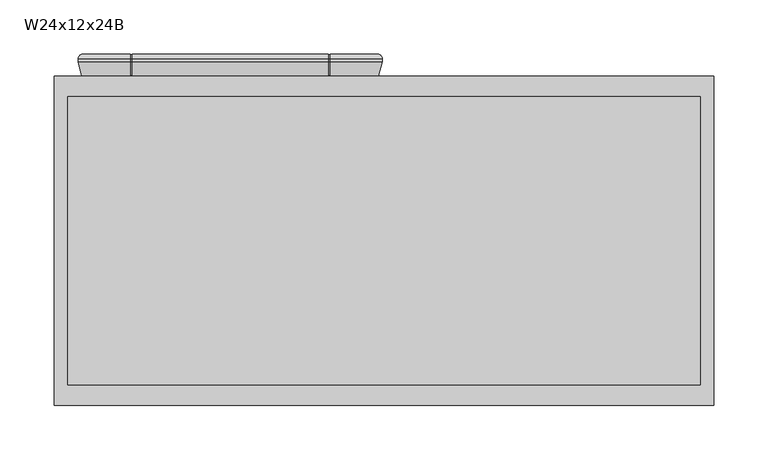
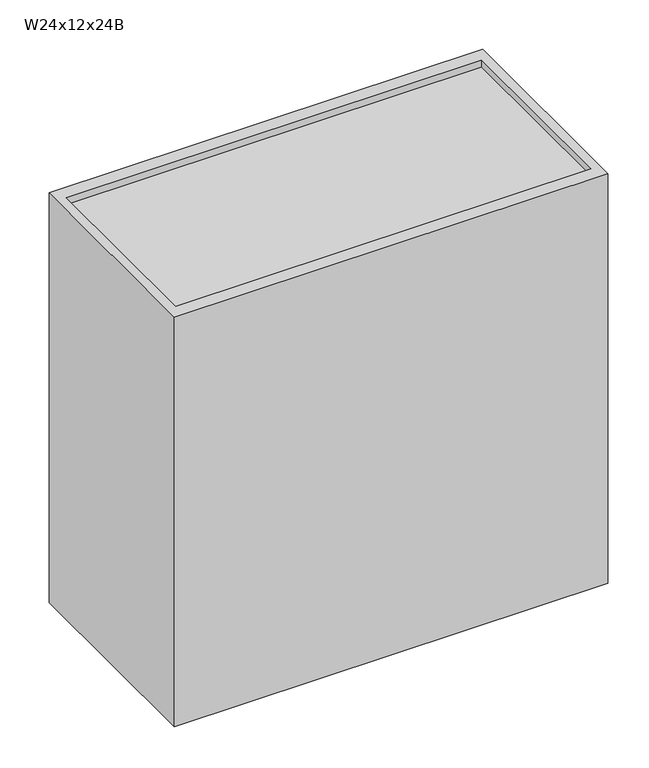
"""IFC4 building model written with IfcOpenShell, lengths in millimetres: furniture geometry, Cabinet-Wall-Merillat-Double_Door-Marlin : W24x12x24B."""

from ifc_helpers import new_model, si_unit, frame, origin, place, context, project, spatial, polyline, circle_curve, ellipse_curve, outline, extrude, faceted_brep, source, transform, mapped, element, save
from ifc_brep_helpers import plane_surface, cylinder_surface, advanced_brep


def w24x12x24b_bf14e69a(model_context):
    return source(origin(), model_context, "Body", "SolidModel", [
        advanced_brep(
        [(-24.0971608, 382.5621, 2108.2), (-21.0006683, 387.0325, 2105.1035075), (-21.0006683, 387.0325, 1552.4964925), (-24.0971608, 382.5621, 1549.4), (-24.0971608, 379.7935, 1549.4), (-24.0971608, 379.7935, 2108.2), (-20.5919608, 366.7125, 1552.9052), (-20.5919608, 366.7125, 2104.6948), (24.104002, 366.7125, 2059.9988372), (24.104002, 366.7125, 1597.6011628), (24.4741337, 367.50625, 1597.9712945), (26.5552927, 371.96931, 1600.0524535), (26.5552927, 371.96931, 2057.5475465), (24.4741337, 367.50625, 2059.6287055), (25.1555233, 374.2094093, 1598.652684), (25.1555233, 374.2094093, 2058.947316), (10.8278392, 374.4595, 1584.325), (10.8278392, 374.4595, 2073.275), (10.8278392, 379.2855, 1584.325), (10.8278392, 379.2855, 2073.275), (25.1555233, 379.5355907, 1598.652684), (25.1555233, 379.5355907, 2058.947316), (26.5552927, 381.77569, 1600.0524535), (26.5552927, 381.77569, 2057.5475465), (24.4741337, 386.23875, 1597.9712945), (24.1068694, 387.0263508, 1597.6040302), (24.104002, 387.0325, 2059.9988372), (24.4741337, 386.23875, 2059.6287055), (24.1068694, 387.0325, 1552.4964925), (24.1068694, 382.5621, 1549.4), (253.7938467, 387.0325, 1552.4964925), (256.8903392, 382.5621, 1549.4), (208.7261206, 382.5621, 1549.4), (208.7261206, 387.0325, 1552.4964925), (25.6943694, 382.5621, 1549.4), (25.6943694, 387.0325, 1552.4964925), (207.1386206, 387.0325, 1552.4964925), (207.1386206, 382.5621, 1549.4), (24.1068694, 379.7935, 1549.4), (256.8903392, 379.7935, 1549.4), (208.7261206, 379.7935, 1549.4), (25.6943694, 379.7935, 1549.4), (207.1386206, 379.7935, 1549.4), (24.1068694, 366.7125, 1552.9052), (253.3851392, 366.7125, 1552.9052), (208.7261206, 366.7125, 1552.9052), (25.6943694, 366.7125, 1552.9052), (207.1386206, 366.7125, 1552.9052), (206.2378857, 371.96931, 1600.0524535), (25.6943694, 367.50625, 1597.9712945), (25.6943694, 366.7125, 1597.6011628), (207.1386206, 366.7125, 1597.6011628), (207.1386206, 367.50625, 1597.9712945), (208.3190448, 367.50625, 1597.9712945), (207.6376552, 374.2094093, 1598.652684), (221.9653392, 374.4595, 1584.325), (221.9653392, 379.2855, 1584.325), (207.6376552, 379.5355907, 1598.652684), (206.2378857, 381.77569, 1600.0524535), (208.3190448, 386.23875, 1597.9712945), (207.1386206, 386.23875, 1597.9712945), (207.1386206, 387.0325, 1597.6011628), (25.6943694, 387.0325, 1597.6011628), (25.6943694, 386.23875, 1597.9712945), (253.7938467, 387.0325, 2105.1035075), (256.8903392, 382.5621, 2108.2), (256.8903392, 379.7935, 2108.2), (253.3851392, 366.7125, 2104.6948), (208.6891765, 366.7125, 1597.6011628), (208.6891765, 366.7125, 2059.9988372), (208.3190448, 367.50625, 2059.6287055), (206.2378857, 371.96931, 2057.5475465), (207.6376552, 374.2094093, 2058.947316), (221.9653392, 374.4595, 2073.275), (221.9653392, 379.2855, 2073.275), (207.6376552, 379.5355907, 2058.947316), (206.2378857, 381.77569, 2057.5475465), (208.3190448, 386.23875, 2059.6287055), (208.6891765, 387.0325, 2059.9988372), (208.6891765, 387.0325, 1597.6011628), (208.7261206, 387.0325, 2105.1035075), (208.7261206, 382.5621, 2108.2), (24.1068694, 382.5621, 2108.2), (24.1068694, 387.0325, 2105.1035075), (207.1386206, 382.5621, 2108.2), (207.1386206, 387.0325, 2105.1035075), (25.6943694, 387.0325, 2105.1035075), (25.6943694, 382.5621, 2108.2), (208.7261206, 379.7935, 2108.2), (24.1068694, 379.7935, 2108.2), (207.1386206, 379.7935, 2108.2), (25.6943694, 379.7935, 2108.2), (208.7261206, 366.7125, 2104.6948), (24.1068694, 366.7125, 2104.6948), (207.1386206, 366.7125, 2104.6948), (25.6943694, 366.7125, 2104.6948), (207.1386206, 366.7125, 2059.9988372), (25.6943694, 366.7125, 2059.9988372), (207.1386206, 367.50625, 2059.6287055), (25.6943694, 367.50625, 2059.6287055), (25.6943694, 386.23875, 2059.6287055), (25.6943694, 387.0325, 2059.9988372), (207.1386206, 387.0325, 2059.9988372), (207.1386206, 386.23875, 2059.6287055), (207.1386206, 367.50625, 2104.0857412), (207.1386206, 379.8980037, 2107.40625), (207.1386206, 382.5621, 2107.40625), (207.1386206, 386.23875, 2104.9526052), (208.7261206, 386.23875, 2059.6287055), (208.7261206, 386.23875, 2104.9526052), (208.7261206, 382.5621, 2107.40625), (208.7261206, 379.8980037, 2107.40625), (208.7261206, 367.50625, 2104.0857412), (208.7261206, 367.50625, 2059.6287055), (24.1068694, 367.50625, 2059.6287055), (24.1068694, 367.50625, 2104.0857412), (24.1068694, 379.8980037, 2107.40625), (24.1068694, 382.5621, 2107.40625), (24.1068694, 386.23875, 2104.9526052), (24.1068694, 386.23875, 2059.6287055), (25.6943694, 386.23875, 2104.9526052), (25.6943694, 382.5621, 2107.40625), (25.6943694, 379.8980037, 2107.40625), (25.6943694, 367.50625, 2104.0857412), (24.1068694, 386.23875, 1597.9712945), (24.1068694, 386.23875, 1552.6473948), (24.1068694, 382.5621, 1550.19375), (24.1068694, 379.8980037, 1550.19375), (24.1068694, 367.50625, 1553.5142588), (24.1068694, 367.50625, 1597.9712945), (25.6943694, 367.50625, 1553.5142588), (25.6943694, 379.8980037, 1550.19375), (25.6943694, 382.5621, 1550.19375), (25.6943694, 386.23875, 1552.6473948), (207.1386206, 386.23875, 1552.6473948), (207.1386206, 382.5621, 1550.19375), (207.1386206, 379.8980037, 1550.19375), (207.1386206, 367.50625, 1553.5142588), (208.7261206, 386.23875, 1597.9712945), (208.7261206, 367.50625, 1597.9712945), (208.7261206, 367.50625, 1553.5142588), (208.7261206, 379.8980037, 1550.19375), (208.7261206, 382.5621, 1550.19375), (208.7261206, 386.23875, 1552.6473948)],
        [
            (0, 1, ellipse_curve(frame((-19.3219608, 382.5621, 2103.4248), z_axis=(-0.7071067811865475, 0.0, -0.7071067811865475), x_axis=(-0.7071067811865474, 0.0, 0.7071067811865476)), 6.7531526, 4.7752)),
            (1, 2),
            (2, 3, ellipse_curve(frame((-19.3219608, 382.5621, 1554.1752), z_axis=(-0.7071067811865475, 0.0, 0.7071067811865475), x_axis=(0.7071067811865474, 0.0, 0.7071067811865476)), 6.7531526, 4.7752)),
            (3, 0),
            (3, 4),
            (4, 5),
            (5, 0),
            (4, 6),
            (6, 7),
            (7, 5),
            (8, 9),
            (9, 10),
            (10, 11),
            (11, 12),
            (12, 13),
            (13, 8),
            (11, 14, ellipse_curve(frame((25.1280392, 372.6348492, 1598.6252), z_axis=(-0.7071067811865475, 0.0, 0.7071067811865475), x_axis=(0.7071067811865474, 0.0, 0.7071067811865476)), 2.2271035, 1.5748)),
            (14, 15),
            (15, 12, ellipse_curve(frame((25.1280392, 372.6348492, 2058.9748), z_axis=(-0.7071067811865475, 0.0, -0.7071067811865475), x_axis=(-0.7071067811865474, 0.0, 0.7071067811865476)), 2.2271035, 1.5748)),
            (14, 16),
            (16, 17),
            (17, 15),
            (16, 18),
            (18, 19),
            (19, 17),
            (18, 20),
            (20, 21),
            (21, 19),
            (20, 22, ellipse_curve(frame((25.1280392, 381.1101508, 1598.6252), z_axis=(-0.7071067811865475, 0.0, 0.7071067811865475), x_axis=(0.7071067811865474, 0.0, 0.7071067811865476)), 2.2271035, 1.5748)),
            (22, 23),
            (23, 21, ellipse_curve(frame((25.1280392, 381.1101508, 2058.9748), z_axis=(-0.7071067811865475, 0.0, -0.7071067811865475), x_axis=(-0.7071067811865474, 0.0, 0.7071067811865476)), 2.2271035, 1.5748)),
            (22, 24),
            (24, 25),
            (25, 26),
            (26, 27),
            (27, 23),
            (2, 28),
            (28, 29, circle_curve(frame((24.1068694, 382.5621, 1554.1752), z_axis=(-1.0, 0.0, 0.0), x_axis=(0.0, -1.0, 0.0)), 4.7752)),
            (29, 3),
            (30, 31, ellipse_curve(frame((252.1151392, 382.5621, 1554.1752), z_axis=(-0.7071067811865475, 0.0, -0.7071067811865475), x_axis=(-0.7071067811865476, 0.0, 0.7071067811865474)), 6.7531526, 4.7752)),
            (31, 32),
            (32, 33, circle_curve(frame((208.7261206, 382.5621, 1554.1752), z_axis=(1.0, 0.0, 0.0), x_axis=(0.0, -1.0, 0.0)), 4.7752)),
            (33, 30),
            (34, 35, circle_curve(frame((25.6943694, 382.5621, 1554.1752), z_axis=(1.0, 0.0, 0.0), x_axis=(0.0, -1.0, 0.0)), 4.7752)),
            (35, 36),
            (36, 37, circle_curve(frame((207.1386206, 382.5621, 1554.1752), z_axis=(-1.0, 0.0, 0.0), x_axis=(0.0, -1.0, 0.0)), 4.7752)),
            (37, 34),
            (29, 38),
            (38, 4),
            (31, 39),
            (39, 40),
            (40, 32),
            (41, 34),
            (37, 42),
            (42, 41),
            (38, 43),
            (43, 6),
            (39, 44),
            (44, 45),
            (45, 40),
            (46, 41),
            (42, 47),
            (47, 46),
            (48, 11),
            (10, 49),
            (49, 50),
            (50, 51),
            (51, 52),
            (52, 53),
            (53, 48),
            (48, 54, ellipse_curve(frame((207.6651392, 372.6348492, 1598.6252), z_axis=(-0.7071067811865475, 0.0, -0.7071067811865475), x_axis=(-0.7071067811865476, 0.0, 0.7071067811865474)), 2.2271035, 1.5748)),
            (54, 14),
            (54, 55),
            (55, 16),
            (55, 56),
            (56, 18),
            (56, 57),
            (57, 20),
            (57, 58, ellipse_curve(frame((207.6651392, 381.1101508, 1598.6252), z_axis=(-0.7071067811865475, 0.0, -0.7071067811865475), x_axis=(-0.7071067811865476, 0.0, 0.7071067811865474)), 2.2271035, 1.5748)),
            (58, 22),
            (58, 59),
            (59, 60),
            (60, 61),
            (61, 62),
            (62, 63),
            (63, 24),
            (30, 64),
            (64, 65, ellipse_curve(frame((252.1151392, 382.5621, 2103.4248), z_axis=(0.7071067811865475, 0.0, -0.7071067811865475), x_axis=(-0.7071067811865474, 0.0, -0.7071067811865476)), 6.7531526, 4.7752)),
            (65, 31),
            (65, 66),
            (66, 39),
            (66, 67),
            (67, 44),
            (68, 69),
            (69, 70),
            (70, 71),
            (71, 48),
            (53, 68),
            (71, 72, ellipse_curve(frame((207.6651392, 372.6348492, 2058.9748), z_axis=(0.7071067811865475, 0.0, -0.7071067811865475), x_axis=(-0.7071067811865474, 0.0, -0.7071067811865476)), 2.2271035, 1.5748)),
            (72, 54),
            (72, 73),
            (73, 55),
            (73, 74),
            (74, 56),
            (74, 75),
            (75, 57),
            (75, 76, ellipse_curve(frame((207.6651392, 381.1101508, 2058.9748), z_axis=(0.7071067811865475, 0.0, -0.7071067811865475), x_axis=(-0.7071067811865474, 0.0, -0.7071067811865476)), 2.2271035, 1.5748)),
            (76, 58),
            (76, 77),
            (77, 78),
            (78, 79),
            (79, 59),
            (64, 80),
            (80, 81, circle_curve(frame((208.7261206, 382.5621, 2103.4248), z_axis=(1.0, 0.0, 0.0), x_axis=(0.0, -1.0, 0.0)), 4.7752)),
            (81, 65),
            (0, 82),
            (82, 83, circle_curve(frame((24.1068694, 382.5621, 2103.4248), z_axis=(-1.0, 0.0, 0.0), x_axis=(0.0, -1.0, 0.0)), 4.7752)),
            (83, 1),
            (84, 85, circle_curve(frame((207.1386206, 382.5621, 2103.4248), z_axis=(-1.0, 0.0, 0.0), x_axis=(0.0, -1.0, 0.0)), 4.7752)),
            (85, 86),
            (86, 87, circle_curve(frame((25.6943694, 382.5621, 2103.4248), z_axis=(1.0, 0.0, 0.0), x_axis=(0.0, -1.0, 0.0)), 4.7752)),
            (87, 84),
            (81, 88),
            (88, 66),
            (5, 89),
            (89, 82),
            (90, 84),
            (87, 91),
            (91, 90),
            (88, 92),
            (92, 67),
            (7, 93),
            (93, 89),
            (94, 90),
            (91, 95),
            (95, 94),
            (43, 9),
            (8, 93),
            (92, 69),
            (68, 45),
            (96, 94),
            (95, 97),
            (97, 96),
            (50, 46),
            (47, 51),
            (12, 71),
            (70, 98),
            (98, 96),
            (97, 99),
            (99, 13),
            (15, 72),
            (17, 73),
            (19, 74),
            (21, 75),
            (23, 76),
            (27, 100),
            (100, 101),
            (101, 102),
            (102, 103),
            (103, 77),
            (83, 26),
            (25, 28),
            (33, 79),
            (78, 80),
            (85, 102),
            (101, 86),
            (35, 62),
            (61, 36),
            (98, 104),
            (104, 105),
            (105, 106),
            (106, 107, circle_curve(frame((207.1386206, 382.5621, 2103.4248), z_axis=(-1.0, 0.0, 0.0), x_axis=(0.0, 0.0, 1.0)), 3.98145)),
            (107, 103),
            (78, 108),
            (108, 109),
            (109, 110, circle_curve(frame((208.7261206, 382.5621, 2103.4248), z_axis=(1.0, 0.0, 0.0), x_axis=(0.0, 0.0, 1.0)), 3.98145)),
            (110, 111),
            (111, 112),
            (112, 113),
            (113, 69),
            (77, 108),
            (107, 109),
            (106, 110),
            (105, 111),
            (104, 112),
            (70, 113),
            (8, 114),
            (114, 115),
            (115, 116),
            (116, 117),
            (117, 118, circle_curve(frame((24.1068694, 382.5621, 2103.4248), z_axis=(-1.0, 0.0, 0.0), x_axis=(0.0, 0.0, 1.0)), 3.98145)),
            (118, 119),
            (119, 26),
            (100, 120),
            (120, 121, circle_curve(frame((25.6943694, 382.5621, 2103.4248), z_axis=(1.0, 0.0, 0.0), x_axis=(0.0, 0.0, 1.0)), 3.98145)),
            (121, 122),
            (122, 123),
            (123, 99),
            (119, 27),
            (118, 120),
            (117, 121),
            (116, 122),
            (115, 123),
            (114, 13),
            (25, 124),
            (124, 125),
            (125, 126, circle_curve(frame((24.1068694, 382.5621, 1554.1752), z_axis=(-1.0, 0.0, 0.0), x_axis=(0.0, 0.0, 1.0)), 3.98145)),
            (126, 127),
            (127, 128),
            (128, 129),
            (129, 9),
            (49, 130),
            (130, 131),
            (131, 132),
            (132, 133, circle_curve(frame((25.6943694, 382.5621, 1554.1752), z_axis=(1.0, 0.0, 0.0), x_axis=(0.0, 0.0, 1.0)), 3.98145)),
            (133, 63),
            (129, 10),
            (128, 130),
            (127, 131),
            (126, 132),
            (125, 133),
            (124, 24),
            (60, 134),
            (134, 135, circle_curve(frame((207.1386206, 382.5621, 1554.1752), z_axis=(-1.0, 0.0, 0.0), x_axis=(0.0, 0.0, 1.0)), 3.98145)),
            (135, 136),
            (136, 137),
            (137, 52),
            (138, 79),
            (68, 139),
            (139, 140),
            (140, 141),
            (141, 142),
            (142, 143, circle_curve(frame((208.7261206, 382.5621, 1554.1752), z_axis=(1.0, 0.0, 0.0), x_axis=(0.0, 0.0, 1.0)), 3.98145)),
            (143, 138),
            (138, 59),
            (53, 139),
            (137, 140),
            (136, 141),
            (135, 142),
            (134, 143),
        ],
        [
            cylinder_surface(frame((-19.3219608, 382.5621, 2108.2), z_axis=(0.0, 0.0, 1.0), x_axis=(0.0, -1.0, 0.0)), 4.7752),
            plane_surface(frame((-24.0971608, 382.5621, 2108.2), z_axis=(-1.0, 0.0, 0.0), x_axis=(0.0, 0.0, -1.0))),
            plane_surface(frame((-24.0971608, 379.7935, 2108.2), z_axis=(-0.9659229350723619, -0.25882983502910506, 0.0), x_axis=(0.0, 0.0, -1.0))),
            plane_surface(frame((24.104002, 366.7125, 2059.9988372), z_axis=(0.9063077870366099, -0.4226182617407856, 0.0), x_axis=(0.0, 0.0, -1.0))),
            cylinder_surface(frame((25.1280392, 372.6348492, 2108.2), z_axis=(0.0, 0.0, 1.0000000000000002), x_axis=(0.01745240643729364, 0.9998476951563912, 0.0)), 1.5748),
            plane_surface(frame((25.1555233, 374.2094093, 2058.947316), z_axis=(0.017452406437322144, 0.9998476951563906, 0.0), x_axis=(0.0, 0.0, -1.0))),
            plane_surface(frame((10.8278392, 374.4595, 2073.275), z_axis=(1.0, 0.0, 0.0), x_axis=(0.0, 0.0, -1.0))),
            plane_surface(frame((10.8278392, 379.2855, 2073.275), z_axis=(0.01745240643727848, -0.9998476951563914, 0.0), x_axis=(0.0, 0.0, -1.0))),
            cylinder_surface(frame((25.1280392, 381.1101508, 2108.2), z_axis=(0.0, 0.0, 1.0000000000000002), x_axis=(0.9063077870367326, 0.42261826174052236, 0.0)), 1.5748),
            plane_surface(frame((26.5552927, 381.77569, 2057.5475465), z_axis=(0.9063077870366333, 0.4226182617407352, 0.0), x_axis=(0.0, 0.0, -1.0))),
            cylinder_surface(frame((-24.0971608, 382.5621, 1554.1752), z_axis=(-1.0, 0.0, 0.0), x_axis=(0.0, -1.0, 0.0)), 4.7752),
            plane_surface(frame((-24.0971608, 382.5621, 1549.4), z_axis=(0.0, 0.0, -1.0), x_axis=(1.0, 0.0, 0.0))),
            plane_surface(frame((-24.0971608, 379.7935, 1549.4), z_axis=(0.0, -0.2588298350291095, -0.9659229350723607), x_axis=(1.0, 0.0, 0.0))),
            plane_surface(frame((24.104002, 366.7125, 1597.6011628), z_axis=(0.0, -0.42261826174078143, 0.9063077870366119), x_axis=(1.0, 0.0, 0.0))),
            cylinder_surface(frame((-24.0971608, 372.6348492, 1598.6252), z_axis=(-1.0000000000000002, 0.0, 0.0), x_axis=(0.0, 0.9998476951563913, 0.017452406437289025)), 1.5748),
            plane_surface(frame((25.1555233, 374.2094093, 1598.652684), z_axis=(0.0, 0.9998476951563907, 0.01745240643731753), x_axis=(1.0, 0.0, 0.0))),
            plane_surface(frame((10.8278392, 374.4595, 1584.325), z_axis=(0.0, 0.0, 1.0), x_axis=(1.0, 0.0, 0.0))),
            plane_surface(frame((10.8278392, 379.2855, 1584.325), z_axis=(0.0, -0.9998476951563913, 0.017452406437283095), x_axis=(1.0, 0.0, 0.0))),
            cylinder_surface(frame((-24.0971608, 381.1101508, 1598.6252), z_axis=(-1.0000000000000002, 0.0, 0.0), x_axis=(0.0, 0.4226182617405265, 0.9063077870367306)), 1.5748),
            plane_surface(frame((26.5552927, 381.77569, 1600.0524535), z_axis=(0.0, 0.4226182617407394, 0.9063077870366314), x_axis=(1.0, 0.0, 0.0))),
            cylinder_surface(frame((252.1151392, 382.5621, 1549.4), z_axis=(0.0, 0.0, -1.0), x_axis=(0.0, -1.0, 0.0)), 4.7752),
            plane_surface(frame((256.8903392, 382.5621, 1549.4), z_axis=(1.0, 0.0, 0.0), x_axis=(0.0, 0.0, 1.0))),
            plane_surface(frame((256.8903392, 379.7935, 1549.4), z_axis=(0.9659229350723619, -0.25882983502910506, 0.0), x_axis=(0.0, 0.0, 1.0))),
            plane_surface(frame((208.6891765, 366.7125, 1597.6011628), z_axis=(-0.9063077870366099, -0.4226182617407856, 0.0), x_axis=(0.0, 0.0, 1.0))),
            cylinder_surface(frame((207.6651392, 372.6348492, 1549.4), z_axis=(0.0, 0.0, -1.0000000000000002), x_axis=(-0.01745240643729364, 0.9998476951563912, 0.0)), 1.5748),
            plane_surface(frame((207.6376552, 374.2094093, 1598.652684), z_axis=(-0.017452406437322144, 0.9998476951563906, 0.0), x_axis=(0.0, 0.0, 1.0))),
            plane_surface(frame((221.9653392, 374.4595, 1584.325), z_axis=(-1.0, 0.0, 0.0), x_axis=(0.0, 0.0, 1.0))),
            plane_surface(frame((221.9653392, 379.2855, 1584.325), z_axis=(-0.01745240643727848, -0.9998476951563914, 0.0), x_axis=(0.0, 0.0, 1.0))),
            cylinder_surface(frame((207.6651392, 381.1101508, 1549.4), z_axis=(0.0, 0.0, -1.0000000000000002), x_axis=(-0.9063077870367326, 0.42261826174052236, 0.0)), 1.5748),
            plane_surface(frame((206.2378857, 381.77569, 1600.0524535), z_axis=(-0.9063077870366333, 0.4226182617407352, 0.0), x_axis=(0.0, 0.0, 1.0))),
            cylinder_surface(frame((256.8903392, 382.5621, 2103.4248), z_axis=(1.0, 0.0, 0.0), x_axis=(0.0, -1.0, 0.0)), 4.7752),
            plane_surface(frame((256.8903392, 382.5621, 2108.2), z_axis=(0.0, 0.0, 1.0), x_axis=(-1.0, 0.0, 0.0))),
            plane_surface(frame((256.8903392, 379.7935, 2108.2), z_axis=(0.0, -0.2588298350291006, 0.9659229350723632), x_axis=(-1.0, 0.0, 0.0))),
            plane_surface(frame((253.3851392, 366.7125, 2104.6948), z_axis=(0.0, -1.0, 0.0), x_axis=(-1.0, 0.0, 0.0))),
            plane_surface(frame((208.6891765, 366.7125, 2059.9988372), z_axis=(0.0, -0.42261826174078976, -0.9063077870366079), x_axis=(-1.0, 0.0, 0.0))),
            cylinder_surface(frame((256.8903392, 372.6348492, 2058.9748), z_axis=(1.0000000000000002, 0.0, 0.0), x_axis=(0.0, 0.999847695156391, -0.017452406437298253)), 1.5748),
            plane_surface(frame((207.6376552, 374.2094093, 2058.947316), z_axis=(0.0, 0.9998476951563905, -0.01745240643732676), x_axis=(-1.0, 0.0, 0.0))),
            plane_surface(frame((221.9653392, 374.4595, 2073.275), z_axis=(0.0, 0.0, -1.0), x_axis=(-1.0, 0.0, 0.0))),
            plane_surface(frame((221.9653392, 379.2855, 2073.275), z_axis=(0.0, -0.9998476951563915, -0.017452406437273867), x_axis=(-1.0, 0.0, 0.0))),
            cylinder_surface(frame((256.8903392, 381.1101508, 2058.9748), z_axis=(1.0000000000000002, 0.0, 0.0), x_axis=(0.0, 0.4226182617405182, -0.9063077870367346)), 1.5748),
            plane_surface(frame((206.2378857, 381.77569, 2057.5475465), z_axis=(0.0, 0.422618261740731, -0.9063077870366353), x_axis=(-1.0, 0.0, 0.0))),
            plane_surface(frame((208.6891765, 387.0325, 2059.9988372), z_axis=(0.0, 1.0, 0.0), x_axis=(-1.0, 0.0, 0.0))),
            plane_surface(frame((207.1386206, 387.0325, 2059.9988372), z_axis=(1.0000000000000002, 0.0, 0.0), x_axis=(0.0, -0.9063077870366395, -0.42261826174072203))),
            plane_surface(frame((208.7261206, 387.0325, 2059.9988372), z_axis=(-1.0000000000000002, 0.0, 0.0), x_axis=(0.0, 0.9063077870366395, 0.42261826174072203))),
            plane_surface(frame((207.1386206, 387.0325, 2059.9988372), z_axis=(0.0, -0.42261826174072203, 0.9063077870366395), x_axis=(1.0, 0.0, 0.0))),
            plane_surface(frame((207.1386206, 386.23875, 2059.6287055), z_axis=(0.0, 1.0, 0.0), x_axis=(1.0, 0.0, 0.0))),
            cylinder_surface(frame((208.7261206, 382.5621, 2103.4248), z_axis=(1.0, 0.0, 0.0), x_axis=(0.0, 0.0, 1.0)), 3.98145),
            plane_surface(frame((207.1386206, 382.5621, 2107.40625), z_axis=(0.0, 0.0, 1.0), x_axis=(1.0, 0.0, 0.0))),
            plane_surface(frame((207.1386206, 379.8980037, 2107.40625), z_axis=(0.0, -0.25882983502916385, 0.9659229350723462), x_axis=(1.0, 0.0, 0.0))),
            plane_surface(frame((207.1386206, 367.50625, 2104.0857412), z_axis=(0.0, -1.0, 0.0), x_axis=(1.0, 0.0, 0.0))),
            plane_surface(frame((207.1386206, 367.50625, 2059.6287055), z_axis=(0.0, 0.4226182617407834, 0.9063077870366109), x_axis=(1.0, 0.0, 0.0))),
            plane_surface(frame((24.1068694, 387.0325, 2059.9988372), z_axis=(1.0, 0.0, 0.0), x_axis=(0.0, -0.9063077870366473, -0.4226182617407054))),
            plane_surface(frame((25.6943694, 387.0325, 2059.9988372), z_axis=(-1.0, 0.0, 0.0), x_axis=(0.0, 0.9063077870366473, 0.4226182617407054))),
            plane_surface(frame((24.1068694, 387.0325, 2059.9988372), z_axis=(0.0, -0.4226182617407054, 0.9063077870366473), x_axis=(1.0, 0.0, 0.0))),
            plane_surface(frame((24.1068694, 386.23875, 2059.6287055), z_axis=(0.0, 1.0, 0.0), x_axis=(1.0, 0.0, 0.0))),
            cylinder_surface(frame((25.6943694, 382.5621, 2103.4248), z_axis=(1.0, 0.0, 0.0), x_axis=(0.0, 0.0, 1.0)), 3.98145),
            plane_surface(frame((24.1068694, 382.5621, 2107.40625), z_axis=(0.0, 0.0, 1.0), x_axis=(1.0, 0.0, 0.0))),
            plane_surface(frame((24.1068694, 379.8980037, 2107.40625), z_axis=(0.0, -0.2588298350291636, 0.9659229350723463), x_axis=(1.0, 0.0, 0.0))),
            plane_surface(frame((24.1068694, 367.50625, 2104.0857412), z_axis=(0.0, -1.0, 0.0), x_axis=(1.0, 0.0, 0.0))),
            plane_surface(frame((24.1068694, 367.50625, 2059.6287055), z_axis=(0.0, 0.4226182617407987, 0.9063077870366038), x_axis=(1.0, 0.0, 0.0))),
            plane_surface(frame((24.1068694, 382.5621, 1558.9504), z_axis=(1.0, 0.0, 0.0), x_axis=(0.0, 1.0, 0.0))),
            plane_surface(frame((25.6943694, 382.5621, 1558.9504), z_axis=(-1.0, 0.0, 0.0), x_axis=(0.0, -1.0, 0.0))),
            plane_surface(frame((24.1068694, 366.7125, 1597.6011628), z_axis=(0.0, 0.42261826174078765, -0.906307787036609), x_axis=(1.0, 0.0, 0.0))),
            plane_surface(frame((24.1068694, 367.50625, 1597.9712945), z_axis=(0.0, -1.0, 0.0), x_axis=(1.0, 0.0, 0.0))),
            plane_surface(frame((24.1068694, 367.50625, 1553.5142588), z_axis=(0.0, -0.25882983502943846, -0.9659229350722726), x_axis=(1.0, 0.0, 0.0))),
            plane_surface(frame((24.1068694, 379.8980037, 1550.19375), z_axis=(0.0, 0.0, -1.0), x_axis=(1.0, 0.0, 0.0))),
            cylinder_surface(frame((25.6943694, 382.5621, 1554.1752), z_axis=(1.0, 0.0, 0.0), x_axis=(0.0, 0.0, 1.0)), 3.98145),
            plane_surface(frame((24.1068694, 386.23875, 1552.6473948), z_axis=(0.0, 1.0, 0.0), x_axis=(1.0, 0.0, 0.0))),
            plane_surface(frame((24.1068694, 386.23875, 1597.9712945), z_axis=(0.0, -0.42261826174073697, -0.9063077870366324), x_axis=(1.0, 0.0, 0.0))),
            plane_surface(frame((207.1386206, 386.23875, 1597.9712945), z_axis=(1.0, 0.0, 0.0), x_axis=(0.0, 0.9063077870366392, -0.4226182617407227))),
            plane_surface(frame((208.7261206, 386.23875, 1597.9712945), z_axis=(-1.0, 0.0, 0.0), x_axis=(0.0, -0.9063077870366392, 0.4226182617407227))),
            plane_surface(frame((207.1386206, 386.23875, 1597.9712945), z_axis=(0.0, -0.4226182617407227, -0.9063077870366392), x_axis=(1.0, 0.0, 0.0))),
            plane_surface(frame((207.1386206, 366.7125, 1597.6011628), z_axis=(0.0, 0.42261826174079387, -0.9063077870366061), x_axis=(1.0, 0.0, 0.0))),
            plane_surface(frame((207.1386206, 367.50625, 1597.9712945), z_axis=(0.0, -1.0, 0.0), x_axis=(1.0, 0.0, 0.0))),
            plane_surface(frame((207.1386206, 367.50625, 1553.5142588), z_axis=(0.0, -0.2588298350294392, -0.9659229350722724), x_axis=(1.0, 0.0, 0.0))),
            plane_surface(frame((207.1386206, 379.8980037, 1550.19375), z_axis=(0.0, 0.0, -1.0), x_axis=(1.0, 0.0, 0.0))),
            cylinder_surface(frame((208.7261206, 382.5621, 1554.1752), z_axis=(1.0, 0.0, 0.0), x_axis=(0.0, 0.0, 1.0)), 3.98145),
            plane_surface(frame((207.1386206, 386.23875, 1552.6473948), z_axis=(0.0, 1.0, 0.0), x_axis=(1.0, 0.0, 0.0))),
        ],
        [
            (0, [[1, 2, 3, 4]]),
            (1, [[-4, 5, 6, 7]]),
            (2, [[-6, 8, 9, 10]]),
            (3, [[11, 12, 13, 14, 15, 16]]),
            (4, [[-14, 17, 18, 19]]),
            (5, [[-18, 20, 21, 22]]),
            (6, [[-21, 23, 24, 25]]),
            (7, [[-24, 26, 27, 28]]),
            (8, [[-27, 29, 30, 31]]),
            (9, [[-30, 32, 33, 34, 35, 36]]),
            (10, [[-3, 37, 38, 39]]),
            (10, [[40, 41, 42, 43]]),
            (10, [[44, 45, 46, 47]]),
            (11, [[-5, -39, 48, 49]]),
            (11, [[50, 51, 52, -41]]),
            (11, [[53, -47, 54, 55]]),
            (12, [[-8, -49, 56, 57]]),
            (12, [[58, 59, 60, -51]]),
            (12, [[61, -55, 62, 63]]),
            (13, [[64, -13, 65, 66, 67, 68, 69, 70]]),
            (14, [[-17, -64, 71, 72]]),
            (15, [[-20, -72, 73, 74]]),
            (16, [[-23, -74, 75, 76]]),
            (17, [[-26, -76, 77, 78]]),
            (18, [[-29, -78, 79, 80]]),
            (19, [[-80, 81, 82, 83, 84, 85, 86, -32]]),
            (20, [[-40, 87, 88, 89]]),
            (21, [[-50, -89, 90, 91]]),
            (22, [[-58, -91, 92, 93]]),
            (23, [[94, 95, 96, 97, -70, 98]]),
            (24, [[-71, -97, 99, 100]]),
            (25, [[-73, -100, 101, 102]]),
            (26, [[-75, -102, 103, 104]]),
            (27, [[-77, -104, 105, 106]]),
            (28, [[-79, -106, 107, 108]]),
            (29, [[-108, 109, 110, 111, 112, -81]]),
            (30, [[-88, 113, 114, 115]]),
            (30, [[-1, 116, 117, 118]]),
            (30, [[119, 120, 121, 122]]),
            (31, [[-90, -115, 123, 124]]),
            (31, [[-7, 125, 126, -116]]),
            (31, [[127, -122, 128, 129]]),
            (32, [[-92, -124, 130, 131]]),
            (32, [[-10, 132, 133, -125]]),
            (32, [[134, -129, 135, 136]]),
            (33, [[-9, -57, 137, -11, 138, -132]]),
            (33, [[-93, -131, 139, -94, 140, -59]]),
            (33, [[141, -136, 142, 143]]),
            (33, [[144, -63, 145, -67]]),
            (34, [[146, -96, 147, 148, -143, 149, 150, -15]]),
            (35, [[-19, 151, -99, -146]]),
            (36, [[-22, 152, -101, -151]]),
            (37, [[-25, 153, -103, -152]]),
            (38, [[-28, 154, -105, -153]]),
            (39, [[-31, 155, -107, -154]]),
            (40, [[-155, -36, 156, 157, 158, 159, 160, -109]]),
            (41, [[-2, -118, 161, -34, 162, -37]]),
            (41, [[-87, -43, 163, -111, 164, -113]]),
            (41, [[165, -158, 166, -120]]),
            (41, [[167, -84, 168, -45]]),
            (42, [[169, 170, 171, 172, 173, -159, -165, -119, -127, -134, -141, -148]]),
            (43, [[174, 175, 176, 177, 178, 179, 180, -139, -130, -123, -114, -164]]),
            (44, [[-174, -110, 181]]),
            (45, [[-173, 182, -175, -181, -160]]),
            (46, [[-172, 183, -176, -182]]),
            (47, [[-171, 184, -177, -183]]),
            (48, [[-170, 185, -178, -184]]),
            (49, [[-169, -147, 186, -179, -185]]),
            (50, [[-180, -186, -95]]),
            (51, [[187, 188, 189, 190, 191, 192, 193, -161, -117, -126, -133, -138]]),
            (52, [[194, 195, 196, 197, 198, -149, -142, -135, -128, -121, -166, -157]]),
            (53, [[-193, 199, -35]]),
            (54, [[-192, 200, -194, -156, -199]]),
            (55, [[-191, 201, -195, -200]]),
            (56, [[-190, 202, -196, -201]]),
            (57, [[-189, 203, -197, -202]]),
            (58, [[-188, 204, -150, -198, -203]]),
            (59, [[-187, -16, -204]]),
            (60, [[205, 206, 207, 208, 209, 210, 211, -137, -56, -48, -38, -162]]),
            (61, [[212, 213, 214, 215, 216, -85, -167, -44, -53, -61, -144, -66]]),
            (62, [[-211, 217, -12]]),
            (63, [[-210, 218, -212, -65, -217]]),
            (64, [[-209, 219, -213, -218]]),
            (65, [[-208, 220, -214, -219]]),
            (66, [[-207, 221, -215, -220]]),
            (67, [[-206, 222, -86, -216, -221]]),
            (68, [[-205, -33, -222]]),
            (69, [[223, 224, 225, 226, 227, -68, -145, -62, -54, -46, -168, -83]]),
            (70, [[228, -163, -42, -52, -60, -140, 229, 230, 231, 232, 233, 234]]),
            (71, [[-228, 235, -112]]),
            (72, [[-229, -98, 236]]),
            (73, [[-227, 237, -230, -236, -69]]),
            (74, [[-226, 238, -231, -237]]),
            (75, [[-225, 239, -232, -238]]),
            (76, [[-224, 240, -233, -239]]),
            (77, [[-223, -82, -235, -234, -240]]),
        ],
    ),
        extrude(outline(polyline([(221.9653392, 379.2855), (221.9653392, 374.4595), (10.8278392, 374.4595), (10.8278392, 379.2855), (221.9653392, 379.2855)])), frame((0.0, 0.0, 1584.325), z_axis=(0.0, 0.0, 1.0), x_axis=(1.0, 0.0, 0.0)), (0.0, 0.0, 1.0), 488.95),
        extrude(outline(polyline([(-8.5711577, 347.6625), (525.0128185, 347.6625), (525.0128185, 80.9625), (-8.5711577, 80.9625), (-8.5711577, 347.6625)])), frame((0.0, 0.0, 1990.725), z_axis=(0.0, 0.0, 1.0), x_axis=(1.0, 0.0, 0.0)), (0.0, 0.0, 1.0), 19.05),
        extrude(outline(polyline([(-8.5711577, 347.6625), (525.0128185, 347.6625), (525.0128185, 80.9625), (-8.5711577, 80.9625), (-8.5711577, 347.6625)])), frame((0.0, 0.0, 1647.825), z_axis=(0.0, 0.0, 1.0), x_axis=(1.0, 0.0, 0.0)), (0.0, 0.0, 1.0), 19.05),
        extrude(outline(polyline([(-8.5711577, 347.6625), (525.0128185, 347.6625), (525.0128185, 80.9625), (-8.5711577, 80.9625), (-8.5711577, 347.6625)])), frame((0.0, 0.0, 1819.275), z_axis=(0.0, 0.0, 1.0), x_axis=(1.0, 0.0, 0.0)), (0.0, 0.0, 1.0), 19.05),
        faceted_brep([(-46.3221608, 61.9125, 2133.6), (-46.3221608, 61.9125, 1524.0), (563.2778392, 61.9125, 1524.0), (563.2778392, 61.9125, 2133.6), (-46.3221608, 366.7125, 2133.6), (563.2778392, 366.7125, 2133.6), (563.2778392, 366.7125, 1524.0), (-46.3221608, 366.7125, 1524.0), (525.0128185, 366.7125, 2095.2735163), (301.9690685, 366.7125, 2095.2735163), (301.9690685, 366.7125, 1561.8672696), (525.0128185, 366.7125, 1561.8672696), (-8.5711577, 366.7125, 2095.2735163), (-8.5711577, 366.7125, 1561.8672696), (214.98661, 366.7125, 1561.8672696), (214.98661, 366.7125, 2095.2735163), (-33.6221608, 80.9625, 1524.0), (550.5778392, 80.9625, 1524.0), (550.5778392, 347.6625, 1524.0), (-33.6221608, 347.6625, 1524.0), (550.5778392, 347.6625, 2133.6), (550.5778392, 80.9625, 2133.6), (-33.6221608, 80.9625, 2133.6), (-33.6221608, 347.6625, 2133.6), (-8.5711577, 80.9625, 2095.2735163), (214.98661, 347.6625, 2095.2735163), (301.9690685, 347.6625, 2095.2735163), (525.0128185, 80.9625, 2095.2735163), (525.0128185, 80.9625, 1561.8672696), (301.9690685, 347.6625, 1561.8672696), (214.98661, 347.6625, 1561.8672696), (-8.5711577, 80.9625, 1561.8672696), (550.5778392, 80.9625, 2122.9851371), (550.5778392, 347.6625, 2122.9851371), (-33.6221608, 347.6625, 2122.9851371), (-33.6221608, 80.9625, 2122.9851371), (-33.6221608, 80.9625, 1533.8352657), (-33.6221608, 347.6625, 1533.8352657), (550.5778392, 347.6625, 1533.8352657), (550.5778392, 80.9625, 1533.8352657)], [[[0, 1, 2, 3]], [[4, 5, 6, 7], [8, 9, 10, 11], [12, 13, 14, 15]], [[1, 0, 4, 7]], [[2, 1, 7, 6], [16, 17, 18, 19]], [[3, 2, 6, 5]], [[0, 3, 5, 4], [20, 21, 22, 23]], [[24, 12, 15, 25, 26, 9, 8, 27]], [[8, 11, 28, 27]], [[28, 11, 10, 29, 30, 14, 13, 31]], [[13, 12, 24, 31]], [[32, 33, 34, 35]], [[33, 32, 21, 20]], [[34, 33, 20, 23]], [[35, 34, 23, 22]], [[32, 35, 22, 21]], [[36, 37, 38, 39]], [[36, 39, 17, 16]], [[39, 38, 18, 17]], [[38, 37, 19, 18]], [[37, 36, 16, 19]], [[24, 27, 28, 31]], [[26, 29, 10, 9]], [[15, 14, 30, 25]], [[29, 26, 25, 30]]]),
    ])


if __name__ == "__main__":
    model = new_model("IFC4")
    model_context = context("Model", 3, world=origin())
    ifc_project = project(units=[si_unit("LENGTHUNIT", "METRE", prefix="MILLI")], contexts=[model_context])
    site = spatial("IfcSite", under=ifc_project)
    building = spatial("IfcBuilding", under=site)
    placement = place(None, origin())
    w24x12x24b_shape = w24x12x24b_bf14e69a(model_context)
    element("IfcFurniture", 1, ObjectType="Cabinet-Wall-Merillat-Double_Door-Marlin : W24x12x24B", at=placement, inside=building, context=model_context, shape_type="MappedRepresentation", body=[
        mapped(w24x12x24b_shape, transform((0.0, 0.0, 0.0), x_axis=(1.0, 0.0, 0.0), y_axis=(0.0, 1.0, 0.0), z_axis=(0.0, 0.0, 1.0))),
    ])
    save(model, "model.ifc")

# Revit data of these elements
# Type "Cabinet-Wall-Merillat-Double_Door-Marlin : W24x12x24B"
#   URL = "https://www.merillat.com/"
#   Product Page URL = "https://www.merillat.com/our-products/"
#   Product Line = "Express"
#   Product Group = "Wall Cabinet"
#   Product Documentation Link = "http://merillatbusiness.com/wp-content/uploads/2014/07/Merillat_Classic_Catalog.pdf"
#   Model = "W2442B"
#   Manufacturer = "Merillat"
#   Height Note = "Actual Height of 21 inches Cabinet is 20 1/2 inches"
#   Glass Door Note = "Glass Cabinet doors are only available in specific sizes. Please refer to the catalog for this information before requesting a glass size."
#   Finish = "Wood"
#   Description = "Wall 2442 Butt Door"
#   Construction Type = "Wall Cabinet"
#   Cabinet Construction Note = "Cabinets with B suffix have BUTT doors without a center frame stile:"
#   Assembly Code = "C1030410"
#   Spacing = 0' - 1"
#   Shelving Height = 0' - 5 1/4"
#   Door Spacing = 0' - 0 1/8"
#   Cabinet Door Width = 0' - 11 1/16"
#   Cabinet Door Height = 1' - 10"
#   Depth = 1' - 0"
#   Height = 2' - 0"
#   Top Of Cabinet = 7' - 0"
#   Width = 2' - 0"
#   COBie.Type = no
#   Top and Bottom Visibility = yes
#   Partial Overlay Butt = yes
#   Partial Overlay = no
#   Number of Shelves Greater than one = 3
#   Number of Shelves = 3
#   Middle Shelf = yes
#   Full Overlay Butt = no
#   Full Overlay = no
#   Elevation Swing Line = yes
#   Door Drawer Material = Wood - Merillat - Pecan(1)
#   Cabinet Material = Wood - Merillat - Pecan(1)
#   Cabinet Door Style = element 806847
# Element 1 (IfcFurniture, "Cabinet-Wall-Merillat-Double_Door-Marlin : W24x12x24B")
#   Materials on its faces: "Wood - Merillat - Pecan(1)"
# Materials
#   "Wood - Merillat - Pecan(1)": class "Wood", colour RGB 108 67 43, transparency 0, Cost = 0
